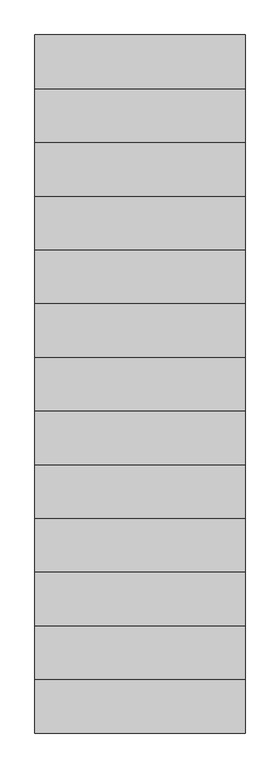
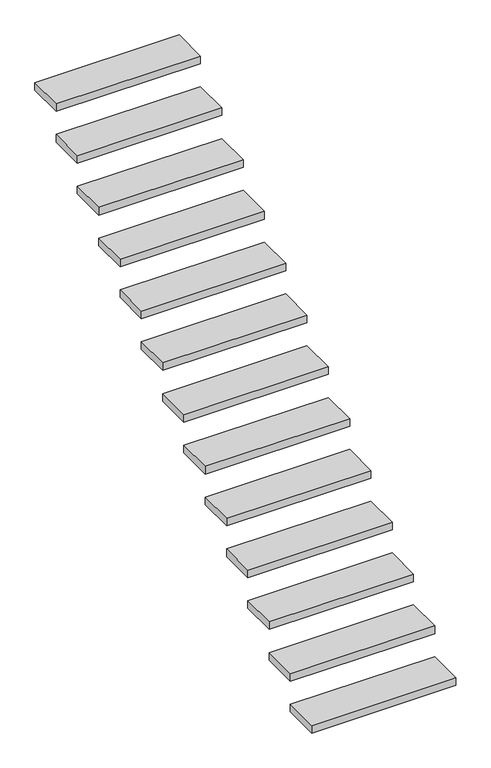
"""IFC4 building model written with IfcOpenShell, lengths in millimetres: stair geometry,   150832 :   150832."""

from ifc_helpers import new_model, si_unit, frame, origin, place, context, project, spatial, polyline, outline, extrude, source, transform, mapped, element, save


def stair_42ef58a3(model_context):
    return source(origin(), model_context, "Body", "SweptSolid", [
        extrude(outline(polyline([(165697.7593015, 42144.7962965), (165697.7593015, 41914.7962965), (164797.7593015, 41914.7962965), (164797.7593015, 42144.7962965), (165697.7593015, 42144.7962965)])), frame((0.0, 0.0, 3482.1428571), z_axis=(0.0, 0.0, 1.0), x_axis=(1.0, 0.0, 0.0)), (0.0, 0.0, 1.0), 50.0),
        extrude(outline(polyline([(165697.7593015, 42374.7962965), (165697.7593015, 42144.7962965), (164797.7593015, 42144.7962965), (164797.7593015, 42374.7962965), (165697.7593015, 42374.7962965)])), frame((0.0, 0.0, 3684.2857143), z_axis=(0.0, 0.0, 1.0), x_axis=(1.0, 0.0, 0.0)), (0.0, 0.0, 1.0), 50.0),
        extrude(outline(polyline([(165697.7593015, 42604.7962965), (165697.7593015, 42374.7962965), (164797.7593015, 42374.7962965), (164797.7593015, 42604.7962965), (165697.7593015, 42604.7962965)])), frame((0.0, 0.0, 3886.4285714), z_axis=(0.0, 0.0, 1.0), x_axis=(1.0, 0.0, 0.0)), (0.0, 0.0, 1.0), 50.0),
        extrude(outline(polyline([(165697.7593015, 42834.7962965), (165697.7593015, 42604.7962965), (164797.7593015, 42604.7962965), (164797.7593015, 42834.7962965), (165697.7593015, 42834.7962965)])), frame((0.0, 0.0, 4088.5714286), z_axis=(0.0, 0.0, 1.0), x_axis=(1.0, 0.0, 0.0)), (0.0, 0.0, 1.0), 50.0),
        extrude(outline(polyline([(165697.7593015, 43064.7962965), (165697.7593015, 42834.7962965), (164797.7593015, 42834.7962965), (164797.7593015, 43064.7962965), (165697.7593015, 43064.7962965)])), frame((0.0, 0.0, 4290.7142857), z_axis=(0.0, 0.0, 1.0), x_axis=(1.0, 0.0, 0.0)), (0.0, 0.0, 1.0), 50.0),
        extrude(outline(polyline([(165697.7593015, 43294.7962965), (165697.7593015, 43064.7962965), (164797.7593015, 43064.7962965), (164797.7593015, 43294.7962965), (165697.7593015, 43294.7962965)])), frame((0.0, 0.0, 4492.8571429), z_axis=(0.0, 0.0, 1.0), x_axis=(1.0, 0.0, 0.0)), (0.0, 0.0, 1.0), 50.0),
        extrude(outline(polyline([(165697.7593015, 43524.7962965), (165697.7593015, 43294.7962965), (164797.7593015, 43294.7962965), (164797.7593015, 43524.7962965), (165697.7593015, 43524.7962965)])), frame((0.0, 0.0, 4695.0), z_axis=(0.0, 0.0, 1.0), x_axis=(1.0, 0.0, 0.0)), (0.0, 0.0, 1.0), 50.0),
        extrude(outline(polyline([(165697.7593015, 43754.7962965), (165697.7593015, 43524.7962965), (164797.7593015, 43524.7962965), (164797.7593015, 43754.7962965), (165697.7593015, 43754.7962965)])), frame((0.0, 0.0, 4897.1428571), z_axis=(0.0, 0.0, 1.0), x_axis=(1.0, 0.0, 0.0)), (0.0, 0.0, 1.0), 50.0),
        extrude(outline(polyline([(165697.7593015, 43984.7962965), (165697.7593015, 43754.7962965), (164797.7593015, 43754.7962965), (164797.7593015, 43984.7962965), (165697.7593015, 43984.7962965)])), frame((0.0, 0.0, 5099.2857143), z_axis=(0.0, 0.0, 1.0), x_axis=(1.0, 0.0, 0.0)), (0.0, 0.0, 1.0), 50.0),
        extrude(outline(polyline([(165697.7593015, 44214.7962965), (165697.7593015, 43984.7962965), (164797.7593015, 43984.7962965), (164797.7593015, 44214.7962965), (165697.7593015, 44214.7962965)])), frame((0.0, 0.0, 5301.4285714), z_axis=(0.0, 0.0, 1.0), x_axis=(1.0, 0.0, 0.0)), (0.0, 0.0, 1.0), 50.0),
        extrude(outline(polyline([(165697.7593015, 44444.7962965), (165697.7593015, 44214.7962965), (164797.7593015, 44214.7962965), (164797.7593015, 44444.7962965), (165697.7593015, 44444.7962965)])), frame((0.0, 0.0, 5503.5714286), z_axis=(0.0, 0.0, 1.0), x_axis=(1.0, 0.0, 0.0)), (0.0, 0.0, 1.0), 50.0),
        extrude(outline(polyline([(165697.7593015, 44674.7962965), (165697.7593015, 44444.7962965), (164797.7593015, 44444.7962965), (164797.7593015, 44674.7962965), (165697.7593015, 44674.7962965)])), frame((0.0, 0.0, 5705.7142857), z_axis=(0.0, 0.0, 1.0), x_axis=(1.0, 0.0, 0.0)), (0.0, 0.0, 1.0), 50.0),
        extrude(outline(polyline([(165697.7593015, 44904.7962965), (165697.7593015, 44674.7962965), (164797.7593015, 44674.7962965), (164797.7593015, 44904.7962965), (165697.7593015, 44904.7962965)])), frame((0.0, 0.0, 5907.8571429), z_axis=(0.0, 0.0, 1.0), x_axis=(1.0, 0.0, 0.0)), (0.0, 0.0, 1.0), 50.0),
    ])


if __name__ == "__main__":
    model = new_model("IFC4")
    model_context = context("Model", 3, world=origin())
    ifc_project = project(units=[si_unit("LENGTHUNIT", "METRE", prefix="MILLI")], contexts=[model_context])
    site = spatial("IfcSite", under=ifc_project)
    building = spatial("IfcBuilding", under=site)
    placement = place(None, origin())
    stair_shape = stair_42ef58a3(model_context)
    element("IfcStair", 1, ObjectType="  150832 :   150832", at=placement, inside=building, context=model_context, shape_type="MappedRepresentation", body=[
        mapped(stair_shape, transform((0.0, 0.0, 0.0), x_axis=(1.0, 0.0, 0.0), y_axis=(0.0, 1.0, 0.0), z_axis=(0.0, 0.0, 1.0))),
    ])
    save(model, "model.ifc")

# Revit data of these elements
# Type "  150832 :   150832"
#   Abrechnungsart = "St"
#   Allright_Bauteil_ID = "0131Tre0659044593"
#   Codetext = "TR-MASSIV-GER\\"
#   Material = "Stahlbeton"
#   Objektname = "Treppe"
#   NameOverride = " "
#   Reference = "STB-Treppe"
#   ThermalTransmittance = 0.0000 BTU/(h·ft²·°F)
#   NosingLength = 0.000 m
#   NumberOfRiser = 14
#   NumberOfTreads = 13
#   RiserHeight = 2.021 m
#   TreadLength = 2.300 m
#   IsExternal = no
#   FireExit = no
#   HandicapAccessible = no
#   HasNonSkidSurface = no
# Element 1 (IfcStair, "  150832 :   150832")
#   Materials on its faces: "weiss"
# Materials
#   "weiss": class "Unassigned", colour RGB 255 255 255, transparency 0
